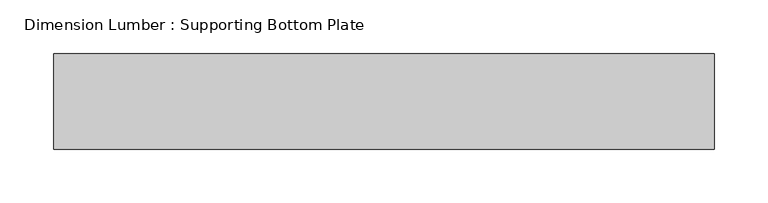
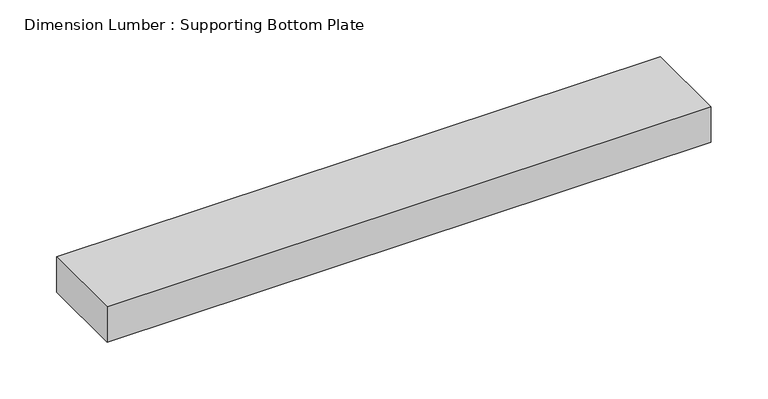
"""IFC4 building model written with IfcOpenShell, lengths in millimetres: beam geometry, Dimension Lumber : Supporting Bottom Plate."""

from ifc_helpers import new_model, si_unit, frame, origin, place, context, project, spatial, polyline, outline, extrude, source, transform, mapped, element, save


def dimension_lumber_supporting_bottom_plate_de809f56(model_context):
    return source(origin(), model_context, "Body", "SweptSolid", [
        extrude(outline(polyline([(160.7438349, 44.45), (160.7438349, -44.45), (-454.81875, -44.45), (-454.81875, 44.45), (160.7438349, 44.45)])), frame((0.0, 0.0, -19.05), z_axis=(0.0, 0.0, 1.0), x_axis=(1.0, 0.0, 0.0)), (0.0, 0.0, 1.0), 38.1),
    ])


if __name__ == "__main__":
    model = new_model("IFC4")
    model_context = context("Model", 3, world=origin())
    ifc_project = project(units=[si_unit("LENGTHUNIT", "METRE", prefix="MILLI")], contexts=[model_context])
    site = spatial("IfcSite", under=ifc_project)
    building = spatial("IfcBuilding", under=site)
    placement = place(None, origin())
    dimension_lumber_supporting_bottom_plate_shape = dimension_lumber_supporting_bottom_plate_de809f56(model_context)
    element("IfcBeam", 1, ObjectType="Dimension Lumber : Supporting Bottom Plate", at=placement, inside=building, context=model_context, shape_type="MappedRepresentation", body=[
        mapped(dimension_lumber_supporting_bottom_plate_shape, transform((0.0, 0.0, 0.0), x_axis=(1.0, 0.0, 0.0), y_axis=(0.0, 1.0, 0.0), z_axis=(0.0, 0.0, 1.0))),
    ])
    save(model, "model.ifc")

# Revit data of these elements
# Type "Dimension Lumber : Supporting Bottom Plate"
#   Assembly Code = "B10"
#   A = 0.0364583 SF
#   Length [instance default] = 5' - 0"
#   b = 0' - 3 1/2"
#   d = 0' - 1 1/2"
#   Structural Material [instance default] = Softwood, Lumber
# Element 1 (IfcBeam, "Dimension Lumber : Supporting Bottom Plate")
#   Structural Material = Douglas Fir #2
#   Materials on its faces: "Douglas Fir #2"
# Materials
#   "Softwood, Lumber": class "Wood", colour RGB 223 192 134, transparency 0, Description = "Pinus Echinata", Cost = 0
#   "Douglas Fir #2": class "Wood", colour RGB 223 192 134, transparency 0, Description = "Pinus Echinata", Cost = 0
